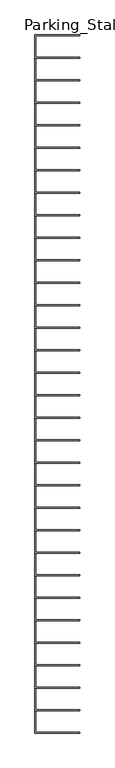
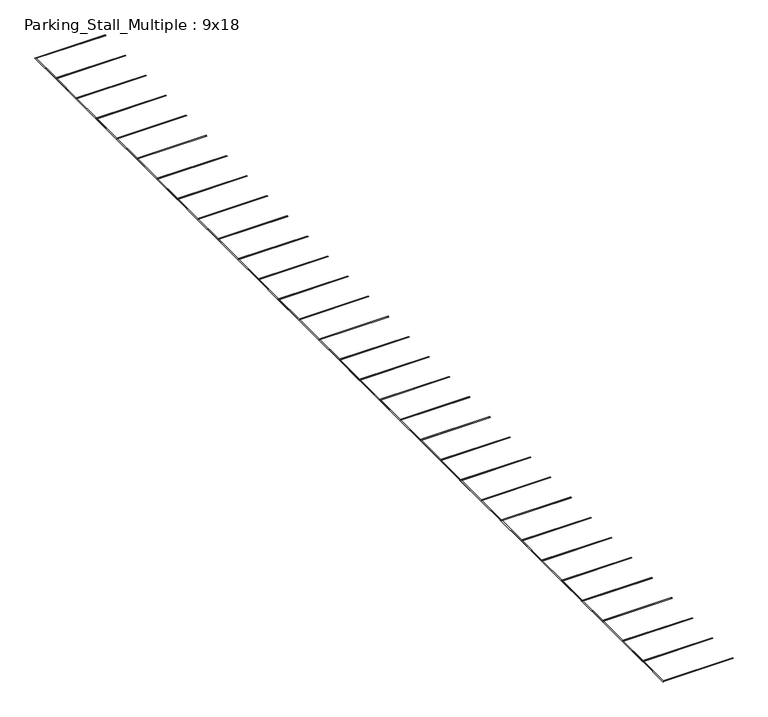
"""IFC4 building model written with IfcOpenShell, lengths in millimetres: proxy geometry, Parking_Stall_Multiple : 9x18."""

import ifcopenshell
import ifcopenshell.guid

model = None  # the IFC model being written
_history = None  # IfcOwnerHistory: only IFC2X3 demands one
_inside = {}  # id of a spatial element -> (the spatial element, [elements in it])
_under = {}  # id of a project, library or spatial element -> (it, [spatial elements below it])
_declared = {}  # id of a project -> (the project, [libraries it declares])
_typed = {}  # id of a type object -> (the type object, [elements of that type])
_made_of = {}  # id of a material, layer set ... -> (it, [elements and type objects made of it])


def new_model(schema):
    """Start an empty IFC model of exactly this schema.

    Asked for "IFC4X3", IfcOpenShell would pick the latest addendum, in which some entities
    have other attributes; the version numbers below select the first issue.
    IFC2X3 requires an IfcOwnerHistory on every rooted entity: one is made here for all.
    """
    global model, _history
    if schema == "IFC4X3":
        model = ifcopenshell.file(schema_version=(4, 3, 0, 0))
    else:
        model = ifcopenshell.file(schema=schema)
    _inside.clear()
    _under.clear()
    _declared.clear()
    _typed.clear()
    _made_of.clear()
    _history = None
    if model.schema == "IFC2X3":
        org = make("IfcOrganization", Name="unknown")
        user = make(
            "IfcPersonAndOrganization",
            ThePerson=make("IfcPerson", FamilyName="unknown"),
            TheOrganization=org,
        )
        app = make(
            "IfcApplication",
            ApplicationDeveloper=org,
            Version="unknown",
            ApplicationFullName="unknown",
            ApplicationIdentifier="unknown",
        )
        _history = make(
            "IfcOwnerHistory",
            OwningUser=user,
            OwningApplication=app,
            ChangeAction="ADDED",
            CreationDate=0,
        )
    return model


def make(cls, **values):
    """One entity of the class cls with the attributes given. An attribute that is None is left unset."""
    return model.create_entity(
        cls, **{name: value for name, value in values.items() if value is not None}
    )


def rooted(cls, **values):
    """An entity with a GlobalId (a new one), such as an element, a storey or a relation."""
    return make(cls, GlobalId=ifcopenshell.guid.new(), OwnerHistory=_history, **values)


def si_unit(unit_type, name, prefix=None):
    """IfcSIUnit, for example si_unit("LENGTHUNIT", "METRE", prefix="MILLI")."""
    return make("IfcSIUnit", UnitType=unit_type, Prefix=prefix, Name=name)


def assignment(units):
    """IfcUnitAssignment: the units of a project."""
    return None if units is None else make("IfcUnitAssignment", Units=units)


def point(xyz):
    """IfcCartesianPoint."""
    return None if xyz is None else make("IfcCartesianPoint", Coordinates=xyz)


def direction(xyz):
    """IfcDirection."""
    return None if xyz is None else make("IfcDirection", DirectionRatios=xyz)


def frame(location, z_axis=None, x_axis=None):
    """IfcAxis2Placement3D, a coordinate frame: its origin and axes. An axis left out is left unset."""
    return make(
        "IfcAxis2Placement3D",
        Location=point(location),
        Axis=direction(z_axis),
        RefDirection=direction(x_axis),
    )


def origin():
    """The frame at (0, 0, 0) with its axes left unset."""
    return frame((0.0, 0.0, 0.0))


def origin_with_axes():
    """The frame at (0, 0, 0) with the z axis (0, 0, 1) and the x axis (1, 0, 0) written out."""
    return frame((0.0, 0.0, 0.0), z_axis=(0.0, 0.0, 1.0), x_axis=(1.0, 0.0, 0.0))


def place(relative_to, where):
    """IfcLocalPlacement: puts the frame where relative to a parent placement (None: the world)."""
    return make(
        "IfcLocalPlacement", PlacementRelTo=relative_to, RelativePlacement=where
    )


def context(
    kind, dimensions, precision=None, world=None, true_north=None, identifier=None
):
    """IfcGeometricRepresentationContext, for example the 3D "Model" context."""
    return make(
        "IfcGeometricRepresentationContext",
        ContextIdentifier=identifier,
        ContextType=kind,
        CoordinateSpaceDimension=dimensions,
        Precision=precision,
        WorldCoordinateSystem=world,
        TrueNorth=true_north,
    )


def project(units=None, contexts=None):
    """IfcProject with its units and contexts."""
    return rooted(
        "IfcProject",
        Name="project",
        RepresentationContexts=contexts,
        UnitsInContext=assignment(units),
    )


def spatial(cls, under=None, at=None, **own):
    """A site, building, storey or space (cls), placed at a placement, below another one or the project."""
    s = rooted(cls, ObjectPlacement=at, **own)
    if under is not None:
        _under.setdefault(under.id(), (under, []))[1].append(s)
    return s


def polyline(points):
    """IfcPolyline through the points."""
    return make("IfcPolyline", Points=[point(p) for p in points])


def outline(outer, holes=None, kind="AREA"):
    """IfcArbitraryClosedProfileDef: a profile drawn as a closed curve; with holes, ...WithVoids."""
    if holes is None:
        return make("IfcArbitraryClosedProfileDef", ProfileType=kind, OuterCurve=outer)
    return make(
        "IfcArbitraryProfileDefWithVoids",
        ProfileType=kind,
        OuterCurve=outer,
        InnerCurves=holes,
    )


def extrude(swept, where, along, depth):
    """IfcExtrudedAreaSolid: the profile swept, set in the frame where, extruded along a direction by depth."""
    return make(
        "IfcExtrudedAreaSolid",
        SweptArea=swept,
        Position=where,
        ExtrudedDirection=direction(along),
        Depth=depth,
    )


def shape(context_of_items, identifier, shape_type, items):
    """IfcShapeRepresentation: the items that make up one representation, for example the "Body"."""
    return make(
        "IfcShapeRepresentation",
        ContextOfItems=context_of_items,
        RepresentationIdentifier=identifier,
        RepresentationType=shape_type,
        Items=items,
    )


def source(mapping_origin, context_of_items, identifier, shape_type, items):
    """IfcRepresentationMap: a shape defined once, which mapped items show again and again."""
    return make(
        "IfcRepresentationMap",
        MappingOrigin=mapping_origin,
        MappedRepresentation=shape(context_of_items, identifier, shape_type, items),
    )


def transform(
    local_origin,
    x_axis=None,
    y_axis=None,
    z_axis=None,
    scale=None,
    scale2=None,
    scale3=None,
    uniform=True,
):
    """IfcCartesianTransformationOperator3D, or its non-uniform kind. x_axis, y_axis, z_axis: its Axis1, 2, 3."""
    if uniform:
        return make(
            "IfcCartesianTransformationOperator3D",
            Axis1=direction(x_axis),
            Axis2=direction(y_axis),
            LocalOrigin=point(local_origin),
            Scale=scale,
            Axis3=direction(z_axis),
        )
    return make(
        "IfcCartesianTransformationOperator3DnonUniform",
        Axis1=direction(x_axis),
        Axis2=direction(y_axis),
        LocalOrigin=point(local_origin),
        Scale=scale,
        Axis3=direction(z_axis),
        Scale2=scale2,
        Scale3=scale3,
    )


def mapped(mapping_source, mapping_target):
    """IfcMappedItem: shows the shape of a source again, moved by a transform."""
    return make(
        "IfcMappedItem", MappingSource=mapping_source, MappingTarget=mapping_target
    )


def made_of(thing, what):
    """Note that an element or type object is made of a material, layer set ...; save() writes the relation."""
    if what is not None:
        _made_of.setdefault(what.id(), (what, []))[1].append(thing)
    return thing


def element(
    cls,
    number,
    at=None,
    inside=None,
    cuts=None,
    type_object=None,
    material=None,
    context=None,
    identifier="Body",
    shape_type=None,
    held_by="IfcProductDefinitionShape",
    body=None,
    shapes=None,
    **own,
):
    """One element of the class cls, such as IfcWall. Its Tag is "e" and its number.

    at: its placement. inside: the storey or other place that contains it. cuts: it is an
    opening in that element (IfcRelVoidsElement). A single representation is given by context,
    identifier, shape_type and body (its items); several are given by shapes. held_by: the class
    of the entity that holds the representations. save() writes the other relations.
    """
    e = rooted(cls, Tag="e%d" % number, ObjectPlacement=at, **own)
    if body is not None:
        shapes = [shape(context, identifier, shape_type, body)]
    if shapes is not None:
        e.Representation = make(held_by, Representations=shapes)
    if inside is not None:
        _inside.setdefault(inside.id(), (inside, []))[1].append(e)
    if cuts is not None:
        rooted(
            "IfcRelVoidsElement", RelatingBuildingElement=cuts, RelatedOpeningElement=e
        )
    if type_object is not None:
        _typed.setdefault(type_object.id(), (type_object, []))[1].append(e)
    return made_of(e, material)


def aggregate(whole, parts):
    """IfcRelAggregates: a whole, such as a stair, and the parts it consists of."""
    return rooted("IfcRelAggregates", RelatingObject=whole, RelatedObjects=parts)


def save(model, path):
    """Write the relations noted so far, then the file.

    IfcRelAggregates (storeys below a building ...), IfcRelContainedInSpatialStructure (elements
    in a storey), IfcRelDefinesByType, IfcRelAssociatesMaterial and IfcRelDeclares: one each for
    every whole, place, type object, material and project.
    """
    for whole, parts in _under.values():
        aggregate(whole, parts)
    for where, things in _inside.values():
        rooted(
            "IfcRelContainedInSpatialStructure",
            RelatedElements=things,
            RelatingStructure=where,
        )
    for kind, things in _typed.values():
        rooted("IfcRelDefinesByType", RelatedObjects=things, RelatingType=kind)
    for what, things in _made_of.values():
        rooted("IfcRelAssociatesMaterial", RelatedObjects=things, RelatingMaterial=what)
    for by, libraries in _declared.values():
        rooted("IfcRelDeclares", RelatingContext=by, RelatedDefinitions=libraries)
    model.write(path)


def parking_stall_multiple_9x18_5371b42e(model_context):
    return source(origin(), model_context, "Body", "SweptSolid", [
        extrude(outline(polyline([(5486.4, 82296.0), (0.0, 82296.0), (0.0, 85115.4), (5486.4, 85115.4), (5486.4, 85039.2), (76.2, 85039.2), (76.2, 82372.2), (5486.4, 82372.2), (5486.4, 82296.0)])), origin_with_axes(), (0.0, 0.0, 1.0), 6.35),
        extrude(outline(polyline([(5486.4, 79552.8), (0.0, 79552.8), (0.0, 82372.2), (5486.4, 82372.2), (5486.4, 82296.0), (76.2, 82296.0), (76.2, 79629.0), (5486.4, 79629.0), (5486.4, 79552.8)])), origin_with_axes(), (0.0, 0.0, 1.0), 6.35),
        extrude(outline(polyline([(5486.4, 76809.6), (0.0, 76809.6), (0.0, 79629.0), (5486.4, 79629.0), (5486.4, 79552.8), (76.2, 79552.8), (76.2, 76885.8), (5486.4, 76885.8), (5486.4, 76809.6)])), origin_with_axes(), (0.0, 0.0, 1.0), 6.35),
        extrude(outline(polyline([(5486.4, 74066.4), (0.0, 74066.4), (0.0, 76885.8), (5486.4, 76885.8), (5486.4, 76809.6), (76.2, 76809.6), (76.2, 74142.6), (5486.4, 74142.6), (5486.4, 74066.4)])), origin_with_axes(), (0.0, 0.0, 1.0), 6.35),
        extrude(outline(polyline([(5486.4, 71323.2), (0.0, 71323.2), (0.0, 74142.6), (5486.4, 74142.6), (5486.4, 74066.4), (76.2, 74066.4), (76.2, 71399.4), (5486.4, 71399.4), (5486.4, 71323.2)])), origin_with_axes(), (0.0, 0.0, 1.0), 6.35),
        extrude(outline(polyline([(5486.4, 68580.0), (0.0, 68580.0), (0.0, 71399.4), (5486.4, 71399.4), (5486.4, 71323.2), (76.2, 71323.2), (76.2, 68656.2), (5486.4, 68656.2), (5486.4, 68580.0)])), origin_with_axes(), (0.0, 0.0, 1.0), 6.35),
        extrude(outline(polyline([(5486.4, 65836.8), (0.0, 65836.8), (0.0, 68656.2), (5486.4, 68656.2), (5486.4, 68580.0), (76.2, 68580.0), (76.2, 65913.0), (5486.4, 65913.0), (5486.4, 65836.8)])), origin_with_axes(), (0.0, 0.0, 1.0), 6.35),
        extrude(outline(polyline([(5486.4, 63093.6), (0.0, 63093.6), (0.0, 65913.0), (5486.4, 65913.0), (5486.4, 65836.8), (76.2, 65836.8), (76.2, 63169.8), (5486.4, 63169.8), (5486.4, 63093.6)])), origin_with_axes(), (0.0, 0.0, 1.0), 6.35),
        extrude(outline(polyline([(5486.4, 60350.4), (0.0, 60350.4), (0.0, 63169.8), (5486.4, 63169.8), (5486.4, 63093.6), (76.2, 63093.6), (76.2, 60426.6), (5486.4, 60426.6), (5486.4, 60350.4)])), origin_with_axes(), (0.0, 0.0, 1.0), 6.35),
        extrude(outline(polyline([(5486.4, 57607.2), (0.0, 57607.2), (0.0, 60426.6), (5486.4, 60426.6), (5486.4, 60350.4), (76.2, 60350.4), (76.2, 57683.4), (5486.4, 57683.4), (5486.4, 57607.2)])), origin_with_axes(), (0.0, 0.0, 1.0), 6.35),
        extrude(outline(polyline([(5486.4, 54864.0), (0.0, 54864.0), (0.0, 57683.4), (5486.4, 57683.4), (5486.4, 57607.2), (76.2, 57607.2), (76.2, 54940.2), (5486.4, 54940.2), (5486.4, 54864.0)])), origin_with_axes(), (0.0, 0.0, 1.0), 6.35),
        extrude(outline(polyline([(5486.4, 52120.8), (0.0, 52120.8), (0.0, 54940.2), (5486.4, 54940.2), (5486.4, 54864.0), (76.2, 54864.0), (76.2, 52197.0), (5486.4, 52197.0), (5486.4, 52120.8)])), origin_with_axes(), (0.0, 0.0, 1.0), 6.35),
        extrude(outline(polyline([(5486.4, 49377.6), (0.0, 49377.6), (0.0, 52197.0), (5486.4, 52197.0), (5486.4, 52120.8), (76.2, 52120.8), (76.2, 49453.8), (5486.4, 49453.8), (5486.4, 49377.6)])), origin_with_axes(), (0.0, 0.0, 1.0), 6.35),
        extrude(outline(polyline([(5486.4, 46634.4), (0.0, 46634.4), (0.0, 49453.8), (5486.4, 49453.8), (5486.4, 49377.6), (76.2, 49377.6), (76.2, 46710.6), (5486.4, 46710.6), (5486.4, 46634.4)])), origin_with_axes(), (0.0, 0.0, 1.0), 6.35),
        extrude(outline(polyline([(5486.4, 43891.2), (0.0, 43891.2), (0.0, 46710.6), (5486.4, 46710.6), (5486.4, 46634.4), (76.2, 46634.4), (76.2, 43967.4), (5486.4, 43967.4), (5486.4, 43891.2)])), origin_with_axes(), (0.0, 0.0, 1.0), 6.35),
        extrude(outline(polyline([(5486.4, 41148.0), (0.0, 41148.0), (0.0, 43967.4), (5486.4, 43967.4), (5486.4, 43891.2), (76.2, 43891.2), (76.2, 41224.2), (5486.4, 41224.2), (5486.4, 41148.0)])), origin_with_axes(), (0.0, 0.0, 1.0), 6.35),
        extrude(outline(polyline([(5486.4, 38404.8), (0.0, 38404.8), (0.0, 41224.2), (5486.4, 41224.2), (5486.4, 41148.0), (76.2, 41148.0), (76.2, 38481.0), (5486.4, 38481.0), (5486.4, 38404.8)])), origin_with_axes(), (0.0, 0.0, 1.0), 6.35),
        extrude(outline(polyline([(5486.4, 35661.6), (0.0, 35661.6), (0.0, 38481.0), (5486.4, 38481.0), (5486.4, 38404.8), (76.2, 38404.8), (76.2, 35737.8), (5486.4, 35737.8), (5486.4, 35661.6)])), origin_with_axes(), (0.0, 0.0, 1.0), 6.35),
        extrude(outline(polyline([(5486.4, 32918.4), (0.0, 32918.4), (0.0, 35737.8), (5486.4, 35737.8), (5486.4, 35661.6), (76.2, 35661.6), (76.2, 32994.6), (5486.4, 32994.6), (5486.4, 32918.4)])), origin_with_axes(), (0.0, 0.0, 1.0), 6.35),
        extrude(outline(polyline([(5486.4, 30175.2), (0.0, 30175.2), (0.0, 32994.6), (5486.4, 32994.6), (5486.4, 32918.4), (76.2, 32918.4), (76.2, 30251.4), (5486.4, 30251.4), (5486.4, 30175.2)])), origin_with_axes(), (0.0, 0.0, 1.0), 6.35),
        extrude(outline(polyline([(5486.4, 27432.0), (0.0, 27432.0), (0.0, 30251.4), (5486.4, 30251.4), (5486.4, 30175.2), (76.2, 30175.2), (76.2, 27508.2), (5486.4, 27508.2), (5486.4, 27432.0)])), origin_with_axes(), (0.0, 0.0, 1.0), 6.35),
        extrude(outline(polyline([(5486.4, 24688.8), (0.0, 24688.8), (0.0, 27508.2), (5486.4, 27508.2), (5486.4, 27432.0), (76.2, 27432.0), (76.2, 24765.0), (5486.4, 24765.0), (5486.4, 24688.8)])), origin_with_axes(), (0.0, 0.0, 1.0), 6.35),
        extrude(outline(polyline([(5486.4, 21945.6), (0.0, 21945.6), (0.0, 24765.0), (5486.4, 24765.0), (5486.4, 24688.8), (76.2, 24688.8), (76.2, 22021.8), (5486.4, 22021.8), (5486.4, 21945.6)])), origin_with_axes(), (0.0, 0.0, 1.0), 6.35),
        extrude(outline(polyline([(5486.4, 19202.4), (0.0, 19202.4), (0.0, 22021.8), (5486.4, 22021.8), (5486.4, 21945.6), (76.2, 21945.6), (76.2, 19278.6), (5486.4, 19278.6), (5486.4, 19202.4)])), origin_with_axes(), (0.0, 0.0, 1.0), 6.35),
        extrude(outline(polyline([(5486.4, 16459.2), (0.0, 16459.2), (0.0, 19278.6), (5486.4, 19278.6), (5486.4, 19202.4), (76.2, 19202.4), (76.2, 16535.4), (5486.4, 16535.4), (5486.4, 16459.2)])), origin_with_axes(), (0.0, 0.0, 1.0), 6.35),
        extrude(outline(polyline([(5486.4, 13716.0), (0.0, 13716.0), (0.0, 16535.4), (5486.4, 16535.4), (5486.4, 16459.2), (76.2, 16459.2), (76.2, 13792.2), (5486.4, 13792.2), (5486.4, 13716.0)])), origin_with_axes(), (0.0, 0.0, 1.0), 6.35),
        extrude(outline(polyline([(5486.4, 10972.8), (0.0, 10972.8), (0.0, 13792.2), (5486.4, 13792.2), (5486.4, 13716.0), (76.2, 13716.0), (76.2, 11049.0), (5486.4, 11049.0), (5486.4, 10972.8)])), origin_with_axes(), (0.0, 0.0, 1.0), 6.35),
        extrude(outline(polyline([(5486.4, 8229.6), (0.0, 8229.6), (0.0, 11049.0), (5486.4, 11049.0), (5486.4, 10972.8), (76.2, 10972.8), (76.2, 8305.8), (5486.4, 8305.8), (5486.4, 8229.6)])), origin_with_axes(), (0.0, 0.0, 1.0), 6.35),
        extrude(outline(polyline([(5486.4, 5486.4), (0.0, 5486.4), (0.0, 8305.8), (5486.4, 8305.8), (5486.4, 8229.6), (76.2, 8229.6), (76.2, 5562.6), (5486.4, 5562.6), (5486.4, 5486.4)])), origin_with_axes(), (0.0, 0.0, 1.0), 6.35),
        extrude(outline(polyline([(5486.4, 2743.2), (0.0, 2743.2), (0.0, 5562.6), (5486.4, 5562.6), (5486.4, 5486.4), (76.2, 5486.4), (76.2, 2819.4), (5486.4, 2819.4), (5486.4, 2743.2)])), origin_with_axes(), (0.0, 0.0, 1.0), 6.35),
        extrude(outline(polyline([(5486.4, 0.0), (0.0, 0.0), (0.0, 2819.4), (5486.4, 2819.4), (5486.4, 2743.2), (76.2, 2743.2), (76.2, 76.2), (5486.4, 76.2), (5486.4, 0.0)])), origin_with_axes(), (0.0, 0.0, 1.0), 6.35),
    ])


if __name__ == "__main__":
    model = new_model("IFC4")
    model_context = context("Model", 3, world=origin())
    ifc_project = project(units=[si_unit("LENGTHUNIT", "METRE", prefix="MILLI")], contexts=[model_context])
    site = spatial("IfcSite", under=ifc_project)
    building = spatial("IfcBuilding", under=site)
    placement = place(None, origin())
    parking_stall_multiple_9x18_shape = parking_stall_multiple_9x18_5371b42e(model_context)
    element("IfcBuildingElementProxy", 1, Name="Parking_Stall_Multiple : 9x18", ObjectType="Parking_Stall_Multiple : 9x18", at=placement, inside=building, context=model_context, shape_type="MappedRepresentation", body=[
        mapped(parking_stall_multiple_9x18_shape, transform((0.0, 0.0, 0.0), x_axis=(1.0, 0.0, 0.0), y_axis=(0.0, 1.0, 0.0), z_axis=(0.0, 0.0, 1.0))),
    ])
    save(model, "model.ifc")

# Revit data of these elements
# Type "Parking_Stall_Multiple : 9x18"
#   Parking_Width_M = 9' - 0"
#   Parking_Run_Length [instance default] = 65' - 0"
#   Parking_Line_Width = 0' - 3"
#   Parking_Length_M = 18' - 0"
#   Single_Parking_Visibility [instance default] = no
#   Parking_ADA_Symbol = no
#   ParkingUnitsArray [instance default] = 7
#   ParkingUnits [instance default] = 7
#   Multiple_Parking_Visibility [instance default] = yes
#   Parking_Line_Material = none
# Element 1 (IfcBuildingElementProxy, "Parking_Stall_Multiple : 9x18")
#   Parking_Run_Length = 281' - 7.51976"
#   ParkingUnitsArray = 31
#   ParkingUnits = 31
